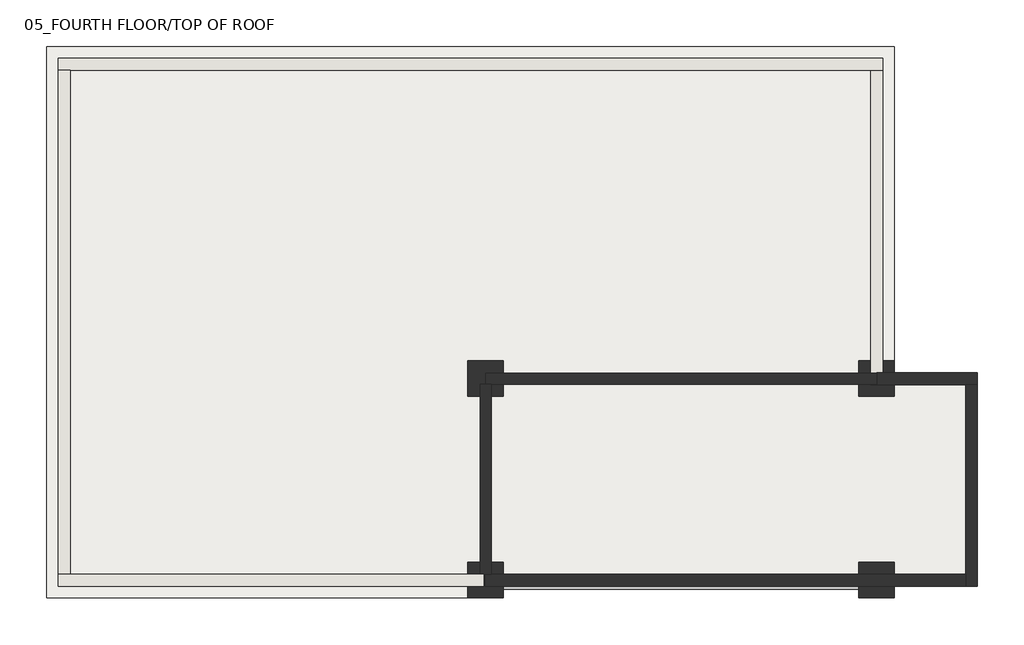
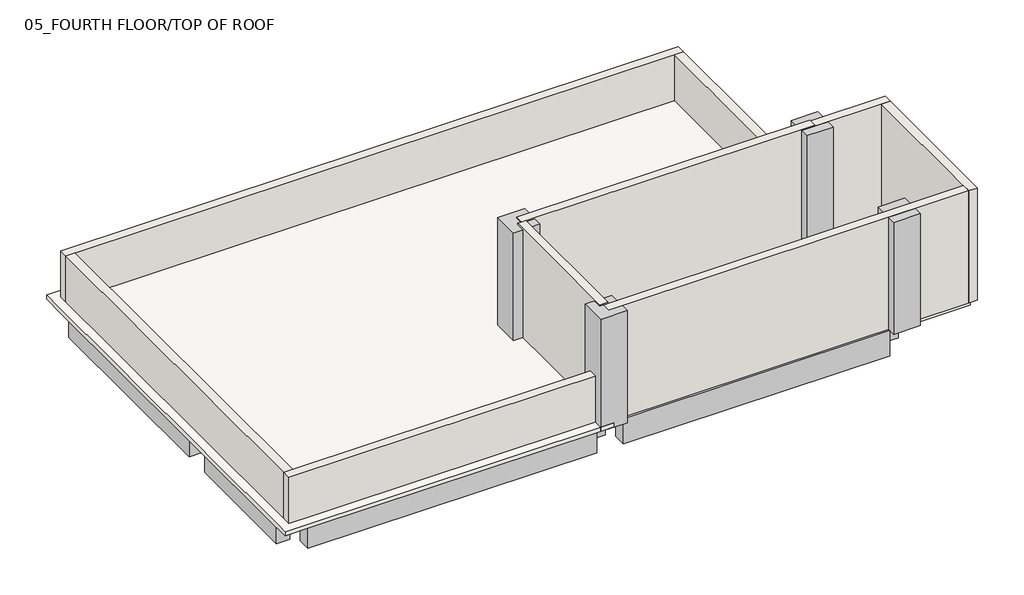
# One storey: 12 beams, 9 walls, 4 columns, 1 roof, 1 slab.
"""IFC4 building model written with IfcOpenShell, lengths in millimetres."""

import ifcopenshell
import ifcopenshell.guid

model = None  # the IFC model being written
_history = None  # IfcOwnerHistory: only IFC2X3 demands one
_inside = {}  # id of a spatial element -> (the spatial element, [elements in it])
_under = {}  # id of a project, library or spatial element -> (it, [spatial elements below it])
_declared = {}  # id of a project -> (the project, [libraries it declares])
_typed = {}  # id of a type object -> (the type object, [elements of that type])
_made_of = {}  # id of a material, layer set ... -> (it, [elements and type objects made of it])


def new_model(schema):
    """Start an empty IFC model of exactly this schema.

    Asked for "IFC4X3", IfcOpenShell would pick the latest addendum, in which some entities
    have other attributes; the version numbers below select the first issue.
    IFC2X3 requires an IfcOwnerHistory on every rooted entity: one is made here for all.
    """
    global model, _history
    if schema == "IFC4X3":
        model = ifcopenshell.file(schema_version=(4, 3, 0, 0))
    else:
        model = ifcopenshell.file(schema=schema)
    _inside.clear()
    _under.clear()
    _declared.clear()
    _typed.clear()
    _made_of.clear()
    _history = None
    if model.schema == "IFC2X3":
        org = make("IfcOrganization", Name="unknown")
        user = make(
            "IfcPersonAndOrganization",
            ThePerson=make("IfcPerson", FamilyName="unknown"),
            TheOrganization=org,
        )
        app = make(
            "IfcApplication",
            ApplicationDeveloper=org,
            Version="unknown",
            ApplicationFullName="unknown",
            ApplicationIdentifier="unknown",
        )
        _history = make(
            "IfcOwnerHistory",
            OwningUser=user,
            OwningApplication=app,
            ChangeAction="ADDED",
            CreationDate=0,
        )
    return model


def make(cls, **values):
    """One entity of the class cls with the attributes given. An attribute that is None is left unset."""
    return model.create_entity(
        cls, **{name: value for name, value in values.items() if value is not None}
    )


def rooted(cls, **values):
    """An entity with a GlobalId (a new one), such as an element, a storey or a relation."""
    return make(cls, GlobalId=ifcopenshell.guid.new(), OwnerHistory=_history, **values)


def si_unit(unit_type, name, prefix=None):
    """IfcSIUnit, for example si_unit("LENGTHUNIT", "METRE", prefix="MILLI")."""
    return make("IfcSIUnit", UnitType=unit_type, Prefix=prefix, Name=name)


def assignment(units):
    """IfcUnitAssignment: the units of a project."""
    return None if units is None else make("IfcUnitAssignment", Units=units)


def point(xyz):
    """IfcCartesianPoint."""
    return None if xyz is None else make("IfcCartesianPoint", Coordinates=xyz)


def direction(xyz):
    """IfcDirection."""
    return None if xyz is None else make("IfcDirection", DirectionRatios=xyz)


def frame(location, z_axis=None, x_axis=None):
    """IfcAxis2Placement3D, a coordinate frame: its origin and axes. An axis left out is left unset."""
    return make(
        "IfcAxis2Placement3D",
        Location=point(location),
        Axis=direction(z_axis),
        RefDirection=direction(x_axis),
    )


def origin():
    """The frame at (0, 0, 0) with its axes left unset."""
    return frame((0.0, 0.0, 0.0))


def place(relative_to, where):
    """IfcLocalPlacement: puts the frame where relative to a parent placement (None: the world)."""
    return make(
        "IfcLocalPlacement", PlacementRelTo=relative_to, RelativePlacement=where
    )


def context(
    kind, dimensions, precision=None, world=None, true_north=None, identifier=None
):
    """IfcGeometricRepresentationContext, for example the 3D "Model" context."""
    return make(
        "IfcGeometricRepresentationContext",
        ContextIdentifier=identifier,
        ContextType=kind,
        CoordinateSpaceDimension=dimensions,
        Precision=precision,
        WorldCoordinateSystem=world,
        TrueNorth=true_north,
    )


def project(units=None, contexts=None):
    """IfcProject with its units and contexts."""
    return rooted(
        "IfcProject",
        Name="project",
        RepresentationContexts=contexts,
        UnitsInContext=assignment(units),
    )


def spatial(cls, under=None, at=None, **own):
    """A site, building, storey or space (cls), placed at a placement, below another one or the project."""
    s = rooted(cls, ObjectPlacement=at, **own)
    if under is not None:
        _under.setdefault(under.id(), (under, []))[1].append(s)
    return s


def polyline(points):
    """IfcPolyline through the points."""
    return make("IfcPolyline", Points=[point(p) for p in points])


def outline(outer, holes=None, kind="AREA"):
    """IfcArbitraryClosedProfileDef: a profile drawn as a closed curve; with holes, ...WithVoids."""
    if holes is None:
        return make("IfcArbitraryClosedProfileDef", ProfileType=kind, OuterCurve=outer)
    return make(
        "IfcArbitraryProfileDefWithVoids",
        ProfileType=kind,
        OuterCurve=outer,
        InnerCurves=holes,
    )


def extrude(swept, where, along, depth):
    """IfcExtrudedAreaSolid: the profile swept, set in the frame where, extruded along a direction by depth."""
    return make(
        "IfcExtrudedAreaSolid",
        SweptArea=swept,
        Position=where,
        ExtrudedDirection=direction(along),
        Depth=depth,
    )


def faces_of(points, faces, orient=None, outer=None):
    """IfcFace entities. A face is a list of loops; a loop is a list of indices into points, from 0.

    orient and outer hold one flag for each loop. By default every Orientation is true, the
    first loop of a face is its IfcFaceOuterBound and the others are IfcFaceBound.
    """
    made = []
    for i, loops in enumerate(faces):
        bounds = []
        for j, loop in enumerate(loops):
            is_outer = j == 0 if outer is None else outer[i][j]
            bounds.append(
                make(
                    "IfcFaceOuterBound" if is_outer else "IfcFaceBound",
                    Bound=make("IfcPolyLoop", Polygon=[points[k] for k in loop]),
                    Orientation=True if orient is None else orient[i][j],
                )
            )
        made.append(make("IfcFace", Bounds=bounds))
    return made


def faceted_brep(points, faces, orient=None, outer=None, voids=None):
    """IfcFacetedBrep: a solid bounded by flat faces; with voids (closed shells), ...WithVoids."""
    shared = [point(p) for p in points]
    hull = make("IfcClosedShell", CfsFaces=faces_of(shared, faces, orient, outer))
    if voids is None:
        return make("IfcFacetedBrep", Outer=hull)
    return make(
        "IfcFacetedBrepWithVoids",
        Outer=hull,
        Voids=[
            make(cls, CfsFaces=faces_of(shared, fs, o, b)) for cls, fs, o, b in voids
        ],
    )


def shape(context_of_items, identifier, shape_type, items):
    """IfcShapeRepresentation: the items that make up one representation, for example the "Body"."""
    return make(
        "IfcShapeRepresentation",
        ContextOfItems=context_of_items,
        RepresentationIdentifier=identifier,
        RepresentationType=shape_type,
        Items=items,
    )


def source(mapping_origin, context_of_items, identifier, shape_type, items):
    """IfcRepresentationMap: a shape defined once, which mapped items show again and again."""
    return make(
        "IfcRepresentationMap",
        MappingOrigin=mapping_origin,
        MappedRepresentation=shape(context_of_items, identifier, shape_type, items),
    )


def transform(
    local_origin,
    x_axis=None,
    y_axis=None,
    z_axis=None,
    scale=None,
    scale2=None,
    scale3=None,
    uniform=True,
):
    """IfcCartesianTransformationOperator3D, or its non-uniform kind. x_axis, y_axis, z_axis: its Axis1, 2, 3."""
    if uniform:
        return make(
            "IfcCartesianTransformationOperator3D",
            Axis1=direction(x_axis),
            Axis2=direction(y_axis),
            LocalOrigin=point(local_origin),
            Scale=scale,
            Axis3=direction(z_axis),
        )
    return make(
        "IfcCartesianTransformationOperator3DnonUniform",
        Axis1=direction(x_axis),
        Axis2=direction(y_axis),
        LocalOrigin=point(local_origin),
        Scale=scale,
        Axis3=direction(z_axis),
        Scale2=scale2,
        Scale3=scale3,
    )


def mapped(mapping_source, mapping_target):
    """IfcMappedItem: shows the shape of a source again, moved by a transform."""
    return make(
        "IfcMappedItem", MappingSource=mapping_source, MappingTarget=mapping_target
    )


def made_of(thing, what):
    """Note that an element or type object is made of a material, layer set ...; save() writes the relation."""
    if what is not None:
        _made_of.setdefault(what.id(), (what, []))[1].append(thing)
    return thing


def element(
    cls,
    number,
    at=None,
    inside=None,
    cuts=None,
    type_object=None,
    material=None,
    context=None,
    identifier="Body",
    shape_type=None,
    held_by="IfcProductDefinitionShape",
    body=None,
    shapes=None,
    **own,
):
    """One element of the class cls, such as IfcWall. Its Tag is "e" and its number.

    at: its placement. inside: the storey or other place that contains it. cuts: it is an
    opening in that element (IfcRelVoidsElement). A single representation is given by context,
    identifier, shape_type and body (its items); several are given by shapes. held_by: the class
    of the entity that holds the representations. save() writes the other relations.
    """
    e = rooted(cls, Tag="e%d" % number, ObjectPlacement=at, **own)
    if body is not None:
        shapes = [shape(context, identifier, shape_type, body)]
    if shapes is not None:
        e.Representation = make(held_by, Representations=shapes)
    if inside is not None:
        _inside.setdefault(inside.id(), (inside, []))[1].append(e)
    if cuts is not None:
        rooted(
            "IfcRelVoidsElement", RelatingBuildingElement=cuts, RelatedOpeningElement=e
        )
    if type_object is not None:
        _typed.setdefault(type_object.id(), (type_object, []))[1].append(e)
    return made_of(e, material)


def aggregate(whole, parts):
    """IfcRelAggregates: a whole, such as a stair, and the parts it consists of."""
    return rooted("IfcRelAggregates", RelatingObject=whole, RelatedObjects=parts)


def save(model, path):
    """Write the relations noted so far, then the file.

    IfcRelAggregates (storeys below a building ...), IfcRelContainedInSpatialStructure (elements
    in a storey), IfcRelDefinesByType, IfcRelAssociatesMaterial and IfcRelDeclares: one each for
    every whole, place, type object, material and project.
    """
    for whole, parts in _under.values():
        aggregate(whole, parts)
    for where, things in _inside.values():
        rooted(
            "IfcRelContainedInSpatialStructure",
            RelatedElements=things,
            RelatingStructure=where,
        )
    for kind, things in _typed.values():
        rooted("IfcRelDefinesByType", RelatedObjects=things, RelatingType=kind)
    for what, things in _made_of.values():
        rooted("IfcRelAssociatesMaterial", RelatedObjects=things, RelatingMaterial=what)
    for by, libraries in _declared.values():
        rooted("IfcRelDeclares", RelatingContext=by, RelatedDefinitions=libraries)
    model.write(path)


def rc_column_rectangular_090fd146(model_context):
    return source(origin(), model_context, "Body", "SweptSolid", [
        extrude(outline(polyline([(300.0, 300.0), (300.0, -300.0), (-300.0, -300.0), (-300.0, 300.0), (300.0, 300.0)])), frame((0.0, 0.0, 11309.9618634), z_axis=(0.0, 0.0, 1.0), x_axis=(1.0, 0.0, 0.0)), (0.0, 0.0, 1.0), 2670.0),
    ])


model = new_model("IFC4")

# Units and contexts
model_context = context("Model", 3, world=origin())
ifc_project = project(units=[si_unit("LENGTHUNIT", "METRE", prefix="MILLI")], contexts=[model_context])

# Site, building, storey
site = spatial("IfcSite", under=ifc_project)
building = spatial("IfcBuilding", under=site)
storey = spatial("IfcBuildingStorey", under=building, Name="05_FOURTH FLOOR/TOP OF ROOF", Elevation=11309.9618634)

# Beams
placement = place(None, origin())
element("IfcBeam", 1, ObjectType="RC Beam_Rectangular : H_SB_AR_S16_B300xH600", at=placement, inside=storey, context=model_context, shape_type="SweptSolid", body=[
    extrude(outline(polyline([(300.0, 1049.5208589), (300.0, 1349.5208589), (6800.0, 1349.5208589), (6800.0, 1049.5208589), (300.0, 1049.5208589)])), frame((0.0, 0.0, 10709.9618634), z_axis=(0.0, 0.0, 1.0), x_axis=(1.0, 0.0, 0.0)), (0.0, 0.0, 1.0), 600.0),
])
element("IfcBeam", 2, ObjectType="RC Beam_Rectangular : H_SB_AR_S16_B300xH600", at=placement, inside=storey, context=model_context, shape_type="SweptSolid", body=[
    extrude(outline(polyline([(7400.0, 1049.5208589), (7400.0, 1349.5208589), (13400.0, 1349.5208589), (13400.0, 1049.5208589), (7400.0, 1049.5208589)])), frame((0.0, 0.0, 10709.9618634), z_axis=(0.0, 0.0, 1.0), x_axis=(1.0, 0.0, 0.0)), (0.0, 0.0, 1.0), 600.0),
])
element("IfcBeam", 3, ObjectType="RC Beam_Rectangular : H_SB_AR_S16_B300xH600", at=placement, inside=storey, context=model_context, shape_type="SweptSolid", body=[
    extrude(outline(polyline([(300.0, 6349.5208589), (300.0, 6649.5208589), (6800.0, 6649.5208589), (6800.0, 6349.5208589), (300.0, 6349.5208589)])), frame((0.0, 0.0, 10709.9618634), z_axis=(0.0, 0.0, 1.0), x_axis=(1.0, 0.0, 0.0)), (0.0, 0.0, 1.0), 600.0),
])
element("IfcBeam", 4, ObjectType="RC Beam_Rectangular : H_SB_AR_S16_B300xH600", at=placement, inside=storey, context=model_context, shape_type="SweptSolid", body=[
    extrude(outline(polyline([(7400.0, 6349.5208589), (7400.0, 6649.5208589), (13400.0, 6649.5208589), (13400.0, 6349.5208589), (7400.0, 6349.5208589)])), frame((0.0, 0.0, 10709.9618634), z_axis=(0.0, 0.0, 1.0), x_axis=(1.0, 0.0, 0.0)), (0.0, 0.0, 1.0), 600.0),
])
element("IfcBeam", 5, ObjectType="RC Beam_Rectangular : H_SB_AR_S16_B300xH600", at=placement, inside=storey, context=model_context, shape_type="SweptSolid", body=[
    extrude(outline(polyline([(300.0, -2350.4791411), (300.0, -2050.4791411), (6800.0, -2050.4791411), (6800.0, -2350.4791411), (300.0, -2350.4791411)])), frame((0.0, 0.0, 10709.9618634), z_axis=(0.0, 0.0, 1.0), x_axis=(1.0, 0.0, 0.0)), (0.0, 0.0, 1.0), 600.0),
])
element("IfcBeam", 6, ObjectType="RC Beam_Rectangular : H_SB_AR_S16_B300xH600", at=placement, inside=storey, context=model_context, shape_type="SweptSolid", body=[
    extrude(outline(polyline([(7400.0, -2350.4791411), (7400.0, -2050.4791411), (13400.0, -2050.4791411), (13400.0, -2350.4791411), (7400.0, -2350.4791411)])), frame((0.0, 0.0, 10709.9618634), z_axis=(0.0, 0.0, 1.0), x_axis=(1.0, 0.0, 0.0)), (0.0, 0.0, 1.0), 600.0),
])
element("IfcBeam", 7, ObjectType="RC Beam_Rectangular : H_SB_AR_S16_B300xH600", at=placement, inside=storey, context=model_context, shape_type="SweptSolid", body=[
    extrude(outline(polyline([(-150.0, 899.5208589), (150.0, 899.5208589), (150.0, -1900.4791411), (-150.0, -1900.4791411), (-150.0, 899.5208589)])), frame((0.0, 0.0, 10709.9618634), z_axis=(0.0, 0.0, 1.0), x_axis=(1.0, 0.0, 0.0)), (0.0, 0.0, 1.0), 600.0),
])
element("IfcBeam", 8, ObjectType="RC Beam_Rectangular : H_SB_AR_S16_B300xH600", at=placement, inside=storey, context=model_context, shape_type="SweptSolid", body=[
    extrude(outline(polyline([(150.0, 1499.5208589), (-150.0, 1499.5208589), (-150.0, 6199.5208589), (150.0, 6199.5208589), (150.0, 1499.5208589)])), frame((0.0, 0.0, 10709.9618634), z_axis=(0.0, 0.0, 1.0), x_axis=(1.0, 0.0, 0.0)), (0.0, 0.0, 1.0), 600.0),
])
element("IfcBeam", 9, ObjectType="RC Beam_Rectangular : H_SB_AR_S16_B300xH600", at=placement, inside=storey, context=model_context, shape_type="SweptSolid", body=[
    extrude(outline(polyline([(6950.0, 899.5208589), (7250.0, 899.5208589), (7250.0, -1900.4791411), (6950.0, -1900.4791411), (6950.0, 899.5208589)])), frame((0.0, 0.0, 10709.9618634), z_axis=(0.0, 0.0, 1.0), x_axis=(1.0, 0.0, 0.0)), (0.0, 0.0, 1.0), 600.0),
])
element("IfcBeam", 10, ObjectType="RC Beam_Rectangular : H_SB_AR_S16_B300xH600", at=placement, inside=storey, context=model_context, shape_type="SweptSolid", body=[
    extrude(outline(polyline([(7250.0, 1499.5208589), (6950.0, 1499.5208589), (6950.0, 6199.5208589), (7250.0, 6199.5208589), (7250.0, 1499.5208589)])), frame((0.0, 0.0, 10709.9618634), z_axis=(0.0, 0.0, 1.0), x_axis=(1.0, 0.0, 0.0)), (0.0, 0.0, 1.0), 600.0),
])
element("IfcBeam", 11, ObjectType="RC Beam_Rectangular : H_SB_AR_S16_B300xH600", at=placement, inside=storey, context=model_context, shape_type="SweptSolid", body=[
    extrude(outline(polyline([(13550.0, 899.5208589), (13850.0, 899.5208589), (13850.0, -1900.4791411), (13550.0, -1900.4791411), (13550.0, 899.5208589)])), frame((0.0, 0.0, 10709.9618634), z_axis=(0.0, 0.0, 1.0), x_axis=(1.0, 0.0, 0.0)), (0.0, 0.0, 1.0), 600.0),
])
element("IfcBeam", 12, ObjectType="RC Beam_Rectangular : H_SB_AR_S16_B300xH600", at=placement, inside=storey, context=model_context, shape_type="SweptSolid", body=[
    extrude(outline(polyline([(13850.0, 1499.5208589), (13550.0, 1499.5208589), (13550.0, 6199.5208589), (13850.0, 6199.5208589), (13850.0, 1499.5208589)])), frame((0.0, 0.0, 10709.9618634), z_axis=(0.0, 0.0, 1.0), x_axis=(1.0, 0.0, 0.0)), (0.0, 0.0, 1.0), 600.0),
])

# Columns
rc_column_rectangular_shape = rc_column_rectangular_090fd146(model_context)
element("IfcColumn", 13, ObjectType="RC_Column_Rectangular : H_SC_AR_S15_W600xL600", at=placement, inside=storey, context=model_context, shape_type="MappedRepresentation", body=[
    mapped(rc_column_rectangular_shape, transform((7100.0, 1199.5208589, 0.0), x_axis=(1.0, 0.0, 0.0), y_axis=(0.0, 1.0, 0.0), z_axis=(0.0, 0.0, 1.0))),
])
element("IfcColumn", 14, ObjectType="RC_Column_Rectangular : H_SC_AR_S15_W600xL600", at=placement, inside=storey, context=model_context, shape_type="MappedRepresentation", body=[
    mapped(rc_column_rectangular_shape, transform((13700.0, 1199.5208589, 0.0), x_axis=(1.0, 0.0, 0.0), y_axis=(0.0, 1.0, 0.0), z_axis=(0.0, 0.0, 1.0))),
])
element("IfcColumn", 15, ObjectType="RC_Column_Rectangular : H_SC_AR_S15_W600xL600", at=placement, inside=storey, context=model_context, shape_type="MappedRepresentation", body=[
    mapped(rc_column_rectangular_shape, transform((13700.0, -2200.4791411, 0.0), x_axis=(1.0, 0.0, 0.0), y_axis=(0.0, 1.0, 0.0), z_axis=(0.0, 0.0, 1.0))),
])
element("IfcColumn", 16, ObjectType="RC_Column_Rectangular : H_SC_AR_S15_W600xL600", at=placement, inside=storey, context=model_context, shape_type="MappedRepresentation", body=[
    mapped(rc_column_rectangular_shape, transform((7100.0, -2200.4791411, 0.0), x_axis=(1.0, 0.0, 0.0), y_axis=(0.0, 1.0, 0.0), z_axis=(0.0, 0.0, 1.0))),
])

# Roof
element("IfcRoof", 17, ObjectType="H_RF_AR_B06_Memb_XPS_PE_Protective Conc", at=placement, inside=storey, context=model_context, shape_type="Brep", body=[
    faceted_brep([(-300.0, 6799.5208589, 11410.9618634), (14000.0, 6799.5208589, 11410.9618634), (14000.0, 6799.5208589, 11309.9618634), (13400.0, 6799.5208589, 11309.9618634), (7400.0, 6799.5208589, 11309.9618634), (6800.0, 6799.5208589, 11309.9618634), (300.0, 6799.5208589, 11309.9618634), (-300.0, 6799.5208589, 11309.9618634), (-300.0, -2500.4791411, 11410.9618634), (-300.0, 6199.5208589, 11309.9618634), (-300.0, 1499.5208589, 11309.9618634), (-300.0, 899.5208589, 11309.9618634), (-300.0, -1900.4791411, 11309.9618634), (-300.0, -2500.4791411, 11309.9618634), (7100.0, -2500.4791411, 11410.9618634), (300.0, -2500.4791411, 11309.9618634), (6800.0, -2500.4791411, 11309.9618634), (7100.0, -2500.4791411, 11309.9618634), (14000.0, 1199.5208589, 11410.9618634), (14000.0, 1199.5208589, 11309.9618634), (14000.0, 1499.5208589, 11309.9618634), (14000.0, 6199.5208589, 11309.9618634), (7100.0, 1199.5208589, 11410.9618634), (7100.0, 1199.5208589, 11309.9618634)], [[[0, 1, 2, 3, 4, 5, 6, 7]], [[8, 0, 7, 9, 10, 11, 12, 13]], [[14, 8, 13, 15, 16, 17]], [[1, 18, 19, 20, 21, 2]], [[18, 22, 23, 19]], [[7, 6, 5, 4, 3, 2, 21, 20, 19, 23, 17, 16, 15, 13, 12, 11, 10, 9]], [[1, 0, 8, 14, 22, 18]], [[22, 14, 17, 23]]]),
])

# Slab
element("IfcSlab", 18, ObjectType="H_FL_AR_S17_RC Slab T150", at=placement, inside=storey, context=model_context, shape_type="SweptSolid", body=[
    extrude(outline(polyline([(15300.0, 1199.5208589), (15300.0, -2200.4791411), (7100.0, -2200.4791411), (7100.0, 1199.5208589), (15300.0, 1199.5208589)])), frame((0.0, 0.0, 11159.9618634), z_axis=(0.0, 0.0, 1.0), x_axis=(1.0, 0.0, 0.0)), (0.0, 0.0, 1.0), 150.0),
])

# Walls
element("IfcWall", 19, ObjectType="H_WA_AR_B02_Ext Wall_RC T200", at=placement, inside=storey, context=model_context, shape_type="Brep", body=[
    faceted_brep([(-100.0, 6399.5208589, 11309.9618634), (100.0, 6399.5208589, 11309.9618634), (13600.0, 6399.5208589, 11309.9618634), (13800.0, 6399.5208589, 11309.9618634), (13800.0, 6399.5208589, 12509.9618634), (13600.0, 6399.5208589, 12509.9618634), (100.0, 6399.5208589, 12509.9618634), (-100.0, 6399.5208589, 12509.9618634), (-100.0, 6599.5208589, 11309.9618634), (-100.0, 6599.5208589, 12509.9618634), (13800.0, 6599.5208589, 12509.9618634), (13800.0, 6599.5208589, 11309.9618634)], [[[0, 1, 2, 3, 4, 5, 6, 7]], [[8, 9, 10, 11]], [[3, 2, 1, 0, 8, 11]], [[7, 6, 5, 4, 10, 9]], [[4, 3, 11, 10]], [[0, 7, 9, 8]]]),
])
element("IfcWall", 20, ObjectType="H_WA_AR_B02_Ext Wall_RC T200", at=placement, inside=storey, context=model_context, shape_type="Brep", body=[
    faceted_brep([(13600.0, 6399.5208589, 11309.9618634), (13600.0, 1286.5208589, 11309.9618634), (13600.0, 1102.5208589, 11309.9618634), (13600.0, 1099.5208589, 11309.9618634), (13600.0, 1099.5208589, 12509.9618634), (13600.0, 1102.5208589, 12509.9618634), (13600.0, 1286.5208589, 12509.9618634), (13600.0, 6399.5208589, 12509.9618634), (13800.0, 6399.5208589, 11309.9618634), (13800.0, 6399.5208589, 12509.9618634), (13800.0, 1299.5208589, 12509.9618634), (13800.0, 1099.5208589, 12509.9618634), (13800.0, 1099.5208589, 11309.9618634), (13800.0, 1299.5208589, 11309.9618634), (13700.0, 1099.5208589, 12509.9618634)], [[[0, 1, 2, 3, 4, 5, 6, 7]], [[8, 9, 10, 11, 12, 13]], [[3, 2, 1, 0, 8, 13, 12]], [[7, 6, 5, 4, 14, 11, 10, 9]], [[0, 7, 9, 8]], [[4, 3, 12, 11, 14]]]),
])
element("IfcWall", 21, ObjectType="H_WA_AR_B02_Ext Wall_RC T200", at=placement, inside=storey, context=model_context, shape_type="Brep", body=[
    faceted_brep([(13800.0, 1099.5208589, 11309.9618634), (15200.0, 1099.5208589, 11309.9618634), (15400.0, 1099.5208589, 11309.9618634), (15400.0, 1099.5208589, 13979.9618634), (15200.0, 1099.5208589, 13979.9618634), (13700.0, 1099.5208589, 13979.9618634), (13700.0, 1099.5208589, 12509.9618634), (13800.0, 1099.5208589, 12509.9618634), (13800.0, 1299.5208589, 11309.9618634), (13800.0, 1299.5208589, 12509.9618634), (13700.0, 1299.5208589, 12509.9618634), (13700.0, 1299.5208589, 13979.9618634), (15400.0, 1299.5208589, 13979.9618634), (15400.0, 1299.5208589, 11309.9618634), (13700.0, 1286.5208589, 12509.9618634), (13700.0, 1102.5208589, 12509.9618634)], [[[0, 1, 2, 3, 4, 5, 6, 7]], [[8, 9, 10, 11, 12, 13]], [[2, 1, 0, 8, 13]], [[5, 4, 3, 12, 11]], [[3, 2, 13, 12]], [[6, 5, 11, 10, 14, 15]], [[6, 15, 14, 10, 9, 7]], [[0, 7, 9, 8]]]),
])
element("IfcWall", 22, ObjectType="H_WA_AR_B02_Ext Wall_RC T200", at=placement, inside=storey, context=model_context, shape_type="Brep", body=[
    faceted_brep([(15200.0, 1099.5208589, 11309.9618634), (15200.0, -2100.4791411, 11309.9618634), (15200.0, -2300.4791411, 11309.9618634), (15200.0, -2300.4791411, 13979.9618634), (15200.0, -2100.4791411, 13979.9618634), (15200.0, 1099.5208589, 13979.9618634), (15400.0, 1099.5208589, 11309.9618634), (15400.0, 1099.5208589, 13979.9618634), (15400.0, -2300.4791411, 13979.9618634), (15400.0, -2300.4791411, 11309.9618634)], [[[0, 1, 2, 3, 4, 5]], [[6, 7, 8, 9]], [[2, 1, 0, 6, 9]], [[5, 4, 3, 8, 7]], [[0, 5, 7, 6]], [[3, 2, 9, 8]]]),
])
element("IfcWall", 23, ObjectType="H_WA_AR_B02_Ext Wall_RC T200", at=placement, inside=storey, context=model_context, shape_type="Brep", body=[
    faceted_brep([(15200.0, -2100.4791411, 11309.9618634), (7197.0, -2100.4791411, 11309.9618634), (7100.0, -2100.4791411, 11309.9618634), (7100.0, -2100.4791411, 13979.9618634), (15200.0, -2100.4791411, 13979.9618634), (15200.0, -2300.4791411, 11309.9618634), (15200.0, -2300.4791411, 13979.9618634), (7100.0, -2300.4791411, 13979.9618634), (7100.0, -2300.4791411, 11309.9618634)], [[[0, 1, 2, 3, 4]], [[5, 6, 7, 8]], [[2, 1, 0, 5, 8]], [[3, 2, 8, 7]], [[4, 3, 7, 6]], [[0, 4, 6, 5]]]),
])
element("IfcWall", 24, ObjectType="H_WA_AR_B02_Ext Wall_RC T200", at=placement, inside=storey, context=model_context, shape_type="SweptSolid", body=[
    extrude(outline(polyline([(100.0, 6399.5208589), (100.0, -2100.4791411), (-100.0, -2100.4791411), (-100.0, 6399.5208589), (100.0, 6399.5208589)])), frame((0.0, 0.0, 11309.9618634), z_axis=(0.0, 0.0, 1.0), x_axis=(1.0, 0.0, 0.0)), (0.0, 0.0, 1.0), 1200.0),
])
element("IfcWall", 25, ObjectType="H_WA_AR_B02_Int Wall_Block T150", at=placement, inside=storey, context=model_context, shape_type="Brep", body=[
    faceted_brep([(7197.0, -2100.4791411, 11309.9618634), (7197.0, 1102.5208589, 11309.9618634), (7197.0, 1102.5208589, 14009.9618634), (7197.0, -2100.4791411, 14009.9618634), (7013.0, -2100.4791411, 11309.9618634), (7013.0, -2100.4791411, 14009.9618634), (7013.0, 1102.5208589, 14009.9618634), (7013.0, 1102.5208589, 11309.9618634), (7100.0, -2100.4791411, 11309.9618634), (7105.0, 1102.5208589, 11309.9618634), (7105.0, 1102.5208589, 14009.9618634)], [[[0, 1, 2, 3]], [[4, 5, 6, 7]], [[1, 0, 8, 4, 7, 9]], [[3, 2, 10, 6, 5]], [[0, 3, 5, 4, 8]], [[2, 1, 9, 7, 6, 10]]]),
])
element("IfcWall", 26, ObjectType="H_WA_AR_B02_Int Wall_Block T150", at=placement, inside=storey, context=model_context, shape_type="Brep", body=[
    faceted_brep([(7105.0, 1102.5208589, 11309.9618634), (7197.0, 1102.5208589, 11309.9618634), (13600.0, 1102.5208589, 11309.9618634), (13600.0, 1102.5208589, 12509.9618634), (13700.0, 1102.5208589, 12509.9618634), (13700.0, 1102.5208589, 14009.9618634), (7197.0, 1102.5208589, 14009.9618634), (7105.0, 1102.5208589, 14009.9618634), (7105.0, 1286.5208589, 11309.9618634), (7105.0, 1286.5208589, 14009.9618634), (13700.0, 1286.5208589, 14009.9618634), (13700.0, 1286.5208589, 12509.9618634), (13600.0, 1286.5208589, 12509.9618634), (13600.0, 1286.5208589, 11309.9618634)], [[[0, 1, 2, 3, 4, 5, 6, 7]], [[8, 9, 10, 11, 12, 13]], [[2, 1, 0, 8, 13]], [[7, 6, 5, 10, 9]], [[0, 7, 9, 8]], [[5, 4, 11, 10]], [[11, 4, 3, 12]], [[3, 2, 13, 12]]]),
])
element("IfcWall", 27, ObjectType="H_WA_AR_B02_Ext Wall_RC T200", at=placement, inside=storey, context=model_context, shape_type="Brep", body=[
    faceted_brep([(7075.0, -2100.4791411, 11309.9618634), (100.0, -2100.4791411, 11309.9618634), (-100.0, -2100.4791411, 11309.9618634), (-100.0, -2100.4791411, 12509.9618634), (100.0, -2100.4791411, 12509.9618634), (7075.0, -2100.4791411, 12509.9618634), (7075.0, -2300.4791411, 11309.9618634), (7075.0, -2300.4791411, 12509.9618634), (-100.0, -2300.4791411, 12509.9618634), (-100.0, -2300.4791411, 11309.9618634)], [[[0, 1, 2, 3, 4, 5]], [[6, 7, 8, 9]], [[2, 1, 0, 6, 9]], [[5, 4, 3, 8, 7]], [[0, 5, 7, 6]], [[3, 2, 9, 8]]]),
])

save(model, "model.ifc")

# Revit data of these elements
# Type "RC Beam_Rectangular : H_SB_AR_S16_B300xH600"
#   중앙부 하부근 = ""
#   중앙부 상부근 = ""
#   중앙부 보조근 = ""
#   중앙부 늑근 = ""
#   외단부 하부근 = ""
#   외단부 상부근 = ""
#   외단부 보조근 = ""
#   외단부 늑근 = ""
#   부호 = "TG3"
#   내단부 하부근 = ""
#   내단부 상부근 = ""
#   내단부 보조근 = ""
#   내단부 늑근 = ""
#   ALL 하부근 = "3-D20"
#   ALL 상부근 = "3-D20"
#   ALL 보조근 = ""
#   ALL 늑근 = "2-D10 @120"
#   Width = 300 mm
#   Height = 600 mm
#   Length [instance default] = 1524 mm
#   b = 300 mm
#   h = 600 mm
#   hec_material3 [instance default] = none
#   hec_material2 [instance default] = none
#   hec_material1 [instance default] = none
#   Structural Material [instance default] = none
#   Assembly Code = ""
# Type "RC_Column_Rectangular : H_SC_AR_S15_W600xL600"
#   Width = 600 mm
#   Length = 600 mm
#   hec_material3 [instance default] = none
#   hec_material2 [instance default] = none
#   hec_material1 [instance default] = none
#   Structural Material [instance default] = none
#   Description = (empty or 0)
# Type "H_RF_AR_B06_Memb_XPS_PE_Protective Conc"
#   Layers, outside or top first: 50 mm no material (function 4); 0 mm no material (function 100); 50 mm no material (function 3); 1 mm no material (function 2)
# Type "H_FL_AR_S17_RC Slab T150"
#   Keynote = ""
#   Type Comments = ""
#   Description = ""
#   Function = 1
#   Layers, outside or top first: 150 mm no material (function 1)
# Type "H_WA_AR_B02_Ext Wall_RC T200"
#   Type Comments = ""
#   Layers, outside or top first: 0 mm no material (function 100); 0 mm no material (function 100); 200 mm no material (function 1); 0 mm no material (function 100); 0 mm no material (function 100); 0 mm no material (function 100)
# Type "H_WA_AR_B02_Int Wall_Block T150"
#   Type Comments = ""
#   Layers, outside or top first: 0 mm no material (function 100); 12 mm no material (function 2); 150 mm no material (function 1); 12 mm no material (function 2); 10 mm no material (function 5)
# Elements 1, 2, 3, 4, 5, 6, 7, 8, 9, 10, 11, 12 (IfcBeam, "RC Beam_Rectangular : H_SB_AR_S16_B300xH600")
#   Comments = ""
#   hec_material3 = none
#   hec_material2 = none
#   hec_material1 = none
#   Structural Material = none
#   Phase Created = New Construction
# Elements 13, 14, 15, 16 (IfcColumn, "RC_Column_Rectangular : H_SC_AR_S15_W600xL600")
#   hec_material3 = none
#   hec_material2 = none
#   hec_material1 = none
#   Structural Material = none
#   Phase Created = New Construction
# Element 17 (IfcRoof, "H_RF_AR_B06_Memb_XPS_PE_Protective Conc")
#   built-in parameter 1001705 = 37.4375 (stored number, unit not read)
#   built-in parameter 1001710 = 33615
#   Phase Created = New Construction
#   Materials on its faces: "Default Roof"
# Element 18 (IfcSlab, "H_FL_AR_S17_RC Slab T150")
#   Height Offset From Level = 0 mm
#   Phase Created = New Construction
#   Materials on its faces: "Default Floor"
# Elements 19, 20, 24, 27 (IfcWall, "H_WA_AR_B02_Ext Wall_RC T200")
#   Top Offset = 0 mm
#   Base Offset = 0 mm
#   Unconnected Height = 1200 mm
#   wall height = 1200 mm
#   Phase Created = New Construction
#   Base Constraint = 05_FOURTH FLOOR/TOP OF ROOF
#   Materials on its faces: "Default Wall"
# Elements 21, 22, 23 (IfcWall, "H_WA_AR_B02_Ext Wall_RC T200")
#   Top Offset = 0 mm
#   Base Offset = 0 mm
#   wall height = 2670 mm
#   Phase Created = New Construction
#   Base Constraint = 05_FOURTH FLOOR/TOP OF ROOF
#   Top Constraint = 06_TOP OF STAIR TOWER ROOF
#   Materials on its faces: "Default Wall"
# Elements 25, 26 (IfcWall, "H_WA_AR_B02_Int Wall_Block T150")
#   Top Offset = 30 mm
#   Base Offset = 0 mm
#   wall height = 2700 mm
#   Phase Created = New Construction
#   Base Constraint = 05_FOURTH FLOOR/TOP OF ROOF
#   Top Constraint = 06_TOP OF STAIR TOWER ROOF
#   Materials on its faces: "Default Wall"
# Materials
#   "Default Roof": class "Miscellaneous", colour RGB 80 80 80, transparency 0
#   "Default Floor": class "Miscellaneous", colour RGB 80 80 80, transparency 0
#   "Default Wall": class "Miscellaneous", colour RGB 80 80 80, transparency 0
# Room at (11043.077, -351.132) mm, phase "New Construction", upper level "06_TOP OF STAIR TOWER ROOF", upper offset 1000 mm, lower offset -1000 mm
#   Comments = ""
#   Number = "145"
#   Name = "STAIRS"
